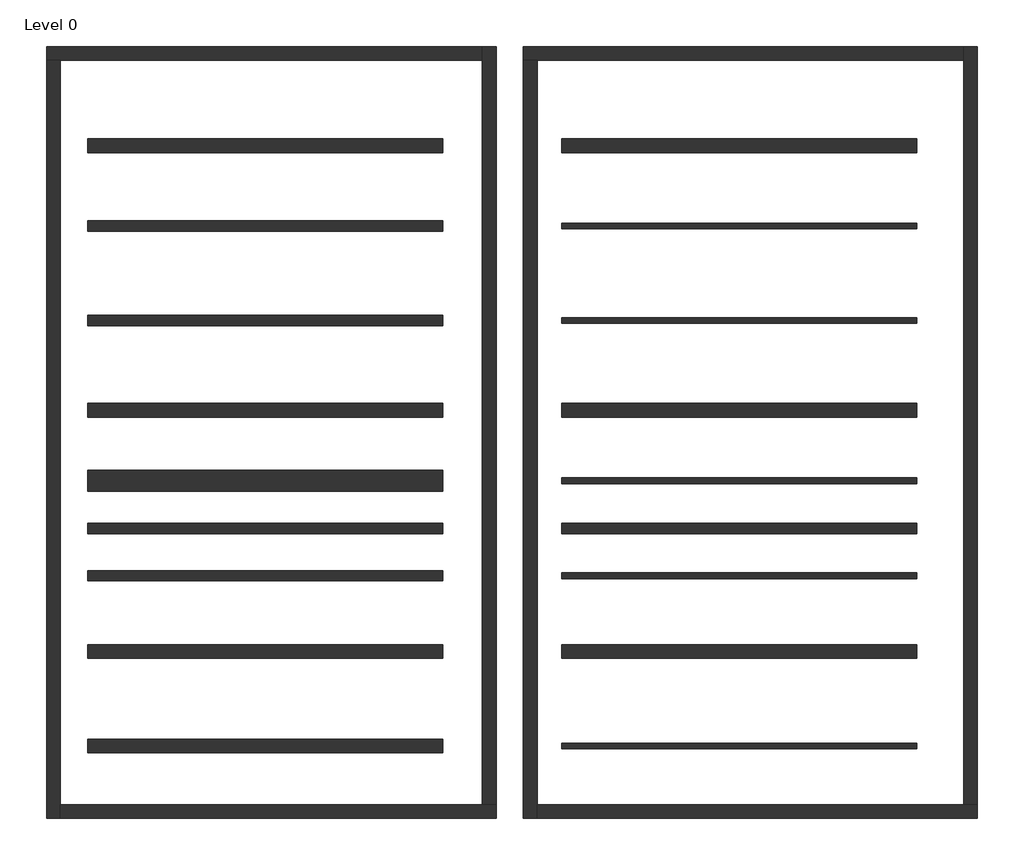
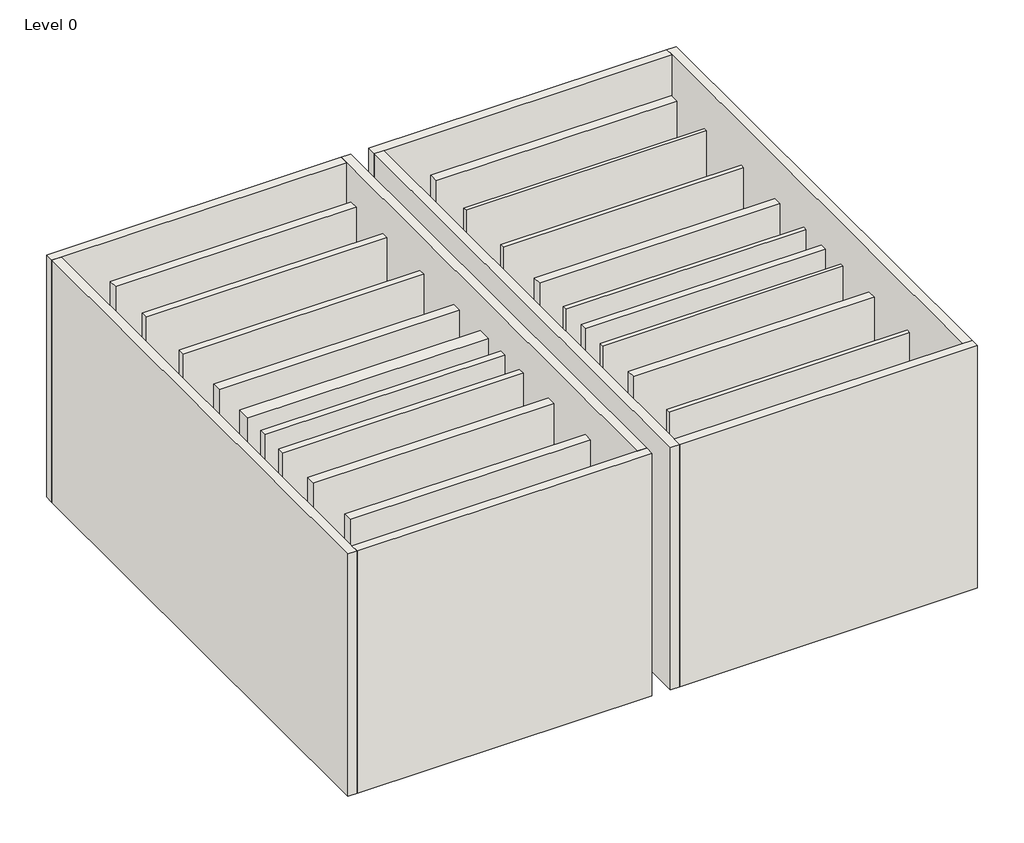
# One storey: 26 walls.
"""IFC4 building model written with IfcOpenShell, lengths in millimetres."""

from ifc_helpers import new_model, si_unit, origin, origin_with_axes, place, context, project, spatial, polyline, outline, extrude, faceted_brep, element, save

model = new_model("IFC4")

# Units and contexts
model_context = context("Model", 3, world=origin())
ifc_project = project(units=[si_unit("LENGTHUNIT", "METRE", prefix="MILLI")], contexts=[model_context])

# Site, building, storey
site = spatial("IfcSite", under=ifc_project)
building = spatial("IfcBuilding", under=site)
storey = spatial("IfcBuildingStorey", under=building, Name="Level 0", Elevation=0.0)

# Walls
placement = place(None, origin())
element("IfcWall", 1, ObjectType="Wall-Ext_102Bwk-75Ins-100LBlk-12P", at=placement, inside=storey, context=model_context, shape_type="SweptSolid", body=[
    extrude(outline(polyline([(-468.4786937, 4696.5247192), (-7968.4786937, 4696.5247192), (-7968.4786937, 4986.5247192), (-468.4786937, 4986.5247192), (-468.4786937, 4696.5247192)])), origin_with_axes(), (0.0, 0.0, 1.0), 8000.0),
])
element("IfcWall", 2, ObjectType="Wall-Ext_102Bwk-75Ins-100LBlk-12P", at=placement, inside=storey, context=model_context, shape_type="SweptSolid", body=[
    extrude(outline(polyline([(-468.4786937, -889.0752808), (-7968.4786937, -889.0752808), (-7968.4786937, -599.0752808), (-468.4786937, -599.0752808), (-468.4786937, -889.0752808)])), origin_with_axes(), (0.0, 0.0, 1.0), 8000.0),
])
element("IfcWall", 3, ObjectType="Wall-Ext_102Bwk-75Ins-100LBlk-12P", at=placement, inside=storey, context=model_context, shape_type="SweptSolid", body=[
    extrude(outline(polyline([(-468.4786937, -5979.4752808), (-7968.4786937, -5979.4752808), (-7968.4786937, -5689.4752808), (-468.4786937, -5689.4752808), (-468.4786937, -5979.4752808)])), origin_with_axes(), (0.0, 0.0, 1.0), 8000.0),
])
element("IfcWall", 4, ObjectType="Wall-Ext_102Bwk-75Ins-100LBlk-12P", at=placement, inside=storey, context=model_context, shape_type="SweptSolid", body=[
    extrude(outline(polyline([(-468.4786937, -7974.6752808), (-7968.4786937, -7974.6752808), (-7968.4786937, -7684.6752808), (-468.4786937, -7684.6752808), (-468.4786937, -7974.6752808)])), origin_with_axes(), (0.0, 0.0, 1.0), 8000.0),
])
element("IfcWall", 5, ObjectType="Wall-Ext_102Bwk-75Ins-100LBlk-12P", at=placement, inside=storey, context=model_context, shape_type="SweptSolid", body=[
    extrude(outline(polyline([(9536.3213063, 4696.5247192), (2036.3213063, 4696.5247192), (2036.3213063, 4986.5247192), (9536.3213063, 4986.5247192), (9536.3213063, 4696.5247192)])), origin_with_axes(), (0.0, 0.0, 1.0), 8000.0),
])
element("IfcWall", 6, ObjectType="Wall-Ext_102Bwk-75Ins-100LBlk-12P", at=placement, inside=storey, context=model_context, shape_type="SweptSolid", body=[
    extrude(outline(polyline([(9536.3213063, -889.0752808), (2036.3213063, -889.0752808), (2036.3213063, -599.0752808), (9536.3213063, -599.0752808), (9536.3213063, -889.0752808)])), origin_with_axes(), (0.0, 0.0, 1.0), 8000.0),
])
element("IfcWall", 7, ObjectType="Wall-Ext_102Bwk-75Ins-100LBlk-12P", at=placement, inside=storey, context=model_context, shape_type="SweptSolid", body=[
    extrude(outline(polyline([(9536.3213063, -5979.4752808), (2036.3213063, -5979.4752808), (2036.3213063, -5689.4752808), (9536.3213063, -5689.4752808), (9536.3213063, -5979.4752808)])), origin_with_axes(), (0.0, 0.0, 1.0), 8000.0),
])
element("IfcWall", 8, ObjectType="Wall-Ext_102Bwk-75Ins-100LBlk-12P", at=placement, inside=storey, context=model_context, shape_type="Brep", body=[
    faceted_brep([(-8835.7862376, 6643.8662444, 0.0), (-8545.7862376, 6643.8662444, 0.0), (364.2137624, 6643.8662444, 0.0), (364.2137624, 6643.8662444, 8000.0), (-8545.7862376, 6643.8662444, 8000.0), (-8835.7862376, 6643.8662444, 8000.0), (-8835.7862376, 6933.8662444, 0.0), (-8835.7862376, 6933.8662444, 8000.0), (364.2137624, 6933.8662444, 8000.0), (364.2137624, 6933.8662444, 0.0)], [[[0, 1, 2, 3, 4, 5]], [[6, 7, 8, 9]], [[2, 1, 0, 6, 9]], [[5, 4, 3, 8, 7]], [[0, 5, 7, 6]], [[3, 2, 9, 8]]]),
])
element("IfcWall", 9, ObjectType="Wall-Ext_102Bwk-75Ins-100LBlk-12P", at=placement, inside=storey, context=model_context, shape_type="Brep", body=[
    faceted_brep([(-8545.7862376, -9356.1337556, 0.0), (-8545.7862376, -9066.1337556, 0.0), (-8545.7862376, 6643.8662444, 0.0), (-8545.7862376, 6643.8662444, 8000.0), (-8545.7862376, -9066.1337556, 8000.0), (-8545.7862376, -9356.1337556, 8000.0), (-8835.7862376, -9356.1337556, 0.0), (-8835.7862376, -9356.1337556, 8000.0), (-8835.7862376, 6643.8662444, 8000.0), (-8835.7862376, 6643.8662444, 0.0)], [[[0, 1, 2, 3, 4, 5]], [[6, 7, 8, 9]], [[2, 1, 0, 6, 9]], [[5, 4, 3, 8, 7]], [[0, 5, 7, 6]], [[3, 2, 9, 8]]]),
])
element("IfcWall", 10, ObjectType="Wall-Ext_102Bwk-75Ins-100LBlk-12P", at=placement, inside=storey, context=model_context, shape_type="Brep", body=[
    faceted_brep([(654.2137624, -9066.1337556, 0.0), (364.2137624, -9066.1337556, 0.0), (-8545.7862376, -9066.1337556, 0.0), (-8545.7862376, -9066.1337556, 8000.0), (364.2137624, -9066.1337556, 8000.0), (654.2137624, -9066.1337556, 8000.0), (654.2137624, -9356.1337556, 0.0), (654.2137624, -9356.1337556, 8000.0), (-8545.7862376, -9356.1337556, 8000.0), (-8545.7862376, -9356.1337556, 0.0)], [[[0, 1, 2, 3, 4, 5]], [[6, 7, 8, 9]], [[2, 1, 0, 6, 9]], [[5, 4, 3, 8, 7]], [[0, 5, 7, 6]], [[3, 2, 9, 8]]]),
])
element("IfcWall", 11, ObjectType="Wall-Ext_102Bwk-75Ins-100LBlk-12P", at=placement, inside=storey, context=model_context, shape_type="Brep", body=[
    faceted_brep([(364.2137624, 6933.8662444, 0.0), (364.2137624, 6643.8662444, 0.0), (364.2137624, -9066.1337556, 0.0), (364.2137624, -9066.1337556, 8000.0), (364.2137624, 6643.8662444, 8000.0), (364.2137624, 6933.8662444, 8000.0), (654.2137624, 6933.8662444, 0.0), (654.2137624, 6933.8662444, 8000.0), (654.2137624, -9066.1337556, 8000.0), (654.2137624, -9066.1337556, 0.0)], [[[0, 1, 2, 3, 4, 5]], [[6, 7, 8, 9]], [[2, 1, 0, 6, 9]], [[5, 4, 3, 8, 7]], [[0, 5, 7, 6]], [[3, 2, 9, 8]]]),
])
element("IfcWall", 12, ObjectType="Wall-Ext_102Bwk-75Ins-100LBlk-12P", at=placement, inside=storey, context=model_context, shape_type="Brep", body=[
    faceted_brep([(1227.1253158, 6643.8662444, 0.0), (1517.1253158, 6643.8662444, 0.0), (10522.526666, 6643.8662444, 0.0), (10522.526666, 6643.8662444, 8000.0), (1517.1253158, 6643.8662444, 8000.0), (1227.1253158, 6643.8662444, 8000.0), (1227.1253158, 6933.8662444, 0.0), (1227.1253158, 6933.8662444, 8000.0), (10522.526666, 6933.8662444, 8000.0), (10522.526666, 6933.8662444, 0.0)], [[[0, 1, 2, 3, 4, 5]], [[6, 7, 8, 9]], [[2, 1, 0, 6, 9]], [[5, 4, 3, 8, 7]], [[0, 5, 7, 6]], [[3, 2, 9, 8]]]),
])
element("IfcWall", 13, ObjectType="Wall-Ext_102Bwk-75Ins-100LBlk-12P", at=placement, inside=storey, context=model_context, shape_type="Brep", body=[
    faceted_brep([(1517.1253158, -9356.1337556, 0.0), (1517.1253158, -9066.1337556, 0.0), (1517.1253158, 6643.8662444, 0.0), (1517.1253158, 6643.8662444, 8000.0), (1517.1253158, -9066.1337556, 8000.0), (1517.1253158, -9356.1337556, 8000.0), (1227.1253158, -9356.1337556, 0.0), (1227.1253158, -9356.1337556, 8000.0), (1227.1253158, 6643.8662444, 8000.0), (1227.1253158, 6643.8662444, 0.0)], [[[0, 1, 2, 3, 4, 5]], [[6, 7, 8, 9]], [[2, 1, 0, 6, 9]], [[5, 4, 3, 8, 7]], [[0, 5, 7, 6]], [[3, 2, 9, 8]]]),
])
element("IfcWall", 14, ObjectType="Wall-Ext_102Bwk-75Ins-100LBlk-12P", at=placement, inside=storey, context=model_context, shape_type="Brep", body=[
    faceted_brep([(10812.526666, -9066.1337556, 0.0), (10522.526666, -9066.1337556, 0.0), (1517.1253158, -9066.1337556, 0.0), (1517.1253158, -9066.1337556, 8000.0), (10522.526666, -9066.1337556, 8000.0), (10812.526666, -9066.1337556, 8000.0), (10812.526666, -9356.1337556, 0.0), (10812.526666, -9356.1337556, 8000.0), (1517.1253158, -9356.1337556, 8000.0), (1517.1253158, -9356.1337556, 0.0)], [[[0, 1, 2, 3, 4, 5]], [[6, 7, 8, 9]], [[2, 1, 0, 6, 9]], [[5, 4, 3, 8, 7]], [[0, 5, 7, 6]], [[3, 2, 9, 8]]]),
])
element("IfcWall", 15, ObjectType="Wall-Ext_102Bwk-75Ins-100LBlk-12P", at=placement, inside=storey, context=model_context, shape_type="Brep", body=[
    faceted_brep([(10522.526666, 6933.8662444, 0.0), (10522.526666, 6643.8662444, 0.0), (10522.526666, -9066.1337556, 0.0), (10522.526666, -9066.1337556, 8000.0), (10522.526666, 6643.8662444, 8000.0), (10522.526666, 6933.8662444, 8000.0), (10812.526666, 6933.8662444, 0.0), (10812.526666, 6933.8662444, 8000.0), (10812.526666, -9066.1337556, 8000.0), (10812.526666, -9066.1337556, 0.0)], [[[0, 1, 2, 3, 4, 5]], [[6, 7, 8, 9]], [[2, 1, 0, 6, 9]], [[5, 4, 3, 8, 7]], [[0, 5, 7, 6]], [[3, 2, 9, 8]]]),
])
element("IfcWall", 16, ObjectType="Wall-Ext_215Bwk", at=placement, inside=storey, context=model_context, shape_type="SweptSolid", body=[
    extrude(outline(polyline([(-468.4786937, 3038.8247192), (-7968.4786937, 3038.8247192), (-7968.4786937, 3253.8247192), (-468.4786937, 3253.8247192), (-468.4786937, 3038.8247192)])), origin_with_axes(), (0.0, 0.0, 1.0), 8000.0),
])
element("IfcWall", 17, ObjectType="Wall-Ext_215Bwk", at=placement, inside=storey, context=model_context, shape_type="SweptSolid", body=[
    extrude(outline(polyline([(-468.4786937, 1043.6247192), (-7968.4786937, 1043.6247192), (-7968.4786937, 1258.6247192), (-468.4786937, 1258.6247192), (-468.4786937, 1043.6247192)])), origin_with_axes(), (0.0, 0.0, 1.0), 8000.0),
])
element("IfcWall", 18, ObjectType="Wall-Ext_215Bwk", at=placement, inside=storey, context=model_context, shape_type="SweptSolid", body=[
    extrude(outline(polyline([(-468.4786937, -3346.7752808), (-7968.4786937, -3346.7752808), (-7968.4786937, -3131.7752808), (-468.4786937, -3131.7752808), (-468.4786937, -3346.7752808)])), origin_with_axes(), (0.0, 0.0, 1.0), 8000.0),
])
element("IfcWall", 19, ObjectType="Wall-Ext_215Bwk", at=placement, inside=storey, context=model_context, shape_type="SweptSolid", body=[
    extrude(outline(polyline([(-468.4786937, -4341.9752808), (-7968.4786937, -4341.9752808), (-7968.4786937, -4126.9752808), (-468.4786937, -4126.9752808), (-468.4786937, -4341.9752808)])), origin_with_axes(), (0.0, 0.0, 1.0), 8000.0),
])
element("IfcWall", 20, ObjectType="Wall-Ext_215Bwk", at=placement, inside=storey, context=model_context, shape_type="SweptSolid", body=[
    extrude(outline(polyline([(9536.3213063, -3346.7752808), (2036.3213063, -3346.7752808), (2036.3213063, -3131.7752808), (9536.3213063, -3131.7752808), (9536.3213063, -3346.7752808)])), origin_with_axes(), (0.0, 0.0, 1.0), 8000.0),
])
element("IfcWall", 21, ObjectType="Wall-Fnd_440Blk", at=placement, inside=storey, context=model_context, shape_type="SweptSolid", body=[
    extrude(outline(polyline([(-468.4786937, -2449.6752808), (-7968.4786937, -2449.6752808), (-7968.4786937, -2009.6752808), (-468.4786937, -2009.6752808), (-468.4786937, -2449.6752808)])), origin_with_axes(), (0.0, 0.0, 1.0), 8000.0),
])
element("IfcWall", 22, ObjectType="Wall-Int_12P-100Blk-12P", at=placement, inside=storey, context=model_context, shape_type="SweptSolid", body=[
    extrude(outline(polyline([(9536.3213063, 3083.8247192), (2036.3213063, 3083.8247192), (2036.3213063, 3208.8247192), (9536.3213063, 3208.8247192), (9536.3213063, 3083.8247192)])), origin_with_axes(), (0.0, 0.0, 1.0), 8000.0),
])
element("IfcWall", 23, ObjectType="Wall-Int_12P-100Blk-12P", at=placement, inside=storey, context=model_context, shape_type="SweptSolid", body=[
    extrude(outline(polyline([(9536.3213063, 1088.6247192), (2036.3213063, 1088.6247192), (2036.3213063, 1213.6247192), (9536.3213063, 1213.6247192), (9536.3213063, 1088.6247192)])), origin_with_axes(), (0.0, 0.0, 1.0), 8000.0),
])
element("IfcWall", 24, ObjectType="Wall-Int_12P-100Blk-12P", at=placement, inside=storey, context=model_context, shape_type="SweptSolid", body=[
    extrude(outline(polyline([(9536.3213063, -7892.1752808), (2036.3213063, -7892.1752808), (2036.3213063, -7767.1752808), (9536.3213063, -7767.1752808), (9536.3213063, -7892.1752808)])), origin_with_axes(), (0.0, 0.0, 1.0), 8000.0),
])
element("IfcWall", 25, ObjectType="Wall-Int_12P-100Blk-12P", at=placement, inside=storey, context=model_context, shape_type="SweptSolid", body=[
    extrude(outline(polyline([(9536.3213063, -4296.9752808), (2036.3213063, -4296.9752808), (2036.3213063, -4171.9752808), (9536.3213063, -4171.9752808), (9536.3213063, -4296.9752808)])), origin_with_axes(), (0.0, 0.0, 1.0), 8000.0),
])
element("IfcWall", 26, ObjectType="Wall-Int_12P-100Blk-12P", at=placement, inside=storey, context=model_context, shape_type="SweptSolid", body=[
    extrude(outline(polyline([(9536.3213063, -2292.1752808), (2036.3213063, -2292.1752808), (2036.3213063, -2167.1752808), (9536.3213063, -2167.1752808), (9536.3213063, -2292.1752808)])), origin_with_axes(), (0.0, 0.0, 1.0), 8000.0),
])

save(model, "model.ifc")

# Revit data of these elements
# Project information
#   Project Issue Date = "Issue Date"
#   Project Status = "Project Status"
#   Client Name = "Owner"
#   Project Address = "Enter address here"
#   Project Name = "Project Name"
#   Project Number = "Project Number"
# Type "Wall-Ext_102Bwk-75Ins-100LBlk-12P"
#   Keynote = "F10"
#   Layers, outside or top first: 102.5 mm "Brick, Common" (function 4); 75 mm "Fiberglass Batt" (function 3); 100 mm "Concrete Masonry Units _Low Density" (function 1); 12.5 mm "Plaster" (function 5)
# Type "Wall-Ext_215Bwk"
#   Keynote = "F10"
#   Layers, outside or top first: 215 mm "Brick, Common" (function 1)
# Type "Wall-Fnd_440Blk"
#   Keynote = "F10"
#   Layers, outside or top first: 440 mm "Concrete Masonry Units" (function 1)
# Type "Wall-Int_12P-100Blk-12P"
#   Layers, outside or top first: 12.5 mm "Plaster" (function 5); 100 mm "Concrete Masonry Units" (function 1); 12.5 mm "Plaster" (function 5)
# Elements 1, 2, 3, 4, 5, 6, 7 (IfcWall, "Wall-Ext_102Bwk-75Ins-100LBlk-12P")
#   Top Offset = 0 mm
#   Base Offset = 0 mm
#   Unconnected Height = 8000 mm
#   wall height = 8000 mm
#   Phase Created = New Construction
#   Base Constraint = Level 0
#   Materials on its faces: "Default Wall", "Plaster", "Brick, Common"
# Elements 8, 9, 10, 11, 12, 13, 14, 15 (IfcWall, "Wall-Ext_102Bwk-75Ins-100LBlk-12P")
#   Top Offset = 0 mm
#   Base Offset = 0 mm
#   Unconnected Height = 8000 mm
#   wall height = 8000 mm
#   Phase Created = New Construction
#   Base Constraint = Level 0
#   Materials on its faces: "Default Wall", "Brick, Common", "Plaster"
# Elements 16, 17, 18, 19, 20 (IfcWall, "Wall-Ext_215Bwk")
#   Top Offset = 0 mm
#   Base Offset = 0 mm
#   Unconnected Height = 8000 mm
#   wall height = 8000 mm
#   Phase Created = New Construction
#   Base Constraint = Level 0
#   Materials on its faces: "Brick, Common"
# Element 21 (IfcWall, "Wall-Fnd_440Blk")
#   Top Offset = 0 mm
#   Base Offset = 0 mm
#   Unconnected Height = 8000 mm
#   wall height = 8000 mm
#   Phase Created = New Construction
#   Base Constraint = Level 0
#   Materials on its faces: "Concrete Masonry Units"
# Elements 22, 23, 24, 25, 26 (IfcWall, "Wall-Int_12P-100Blk-12P")
#   Top Offset = 0 mm
#   Base Offset = 0 mm
#   Unconnected Height = 8000 mm
#   wall height = 8000 mm
#   Phase Created = New Construction
#   Base Constraint = Level 0
#   Materials on its faces: "Default Wall", "Plaster"
# Materials
#   "Brick, Common": class "Masonry", colour RGB 170 100 105, transparency 0, Description = "Common brick", Cost = 0
#   "Fiberglass Batt": class "Generic", colour RGB 127 127 127, transparency 0, Description = "Fiberglass batt insulation", Cost = 0
#   "Concrete Masonry Units _Low Density": class "Masonry", colour RGB 181 181 181, transparency 0, Description = "Concrete masonry units", Cost = 0
#   "Plaster": class "Generic", colour RGB 249 249 249, transparency 0, Description = "Plaster", Cost = 0
#   "Concrete Masonry Units": class "Masonry", colour RGB 181 181 181, transparency 0, Description = "Concrete masonry units", Cost = 0
#   "Default Wall": class "Miscellaneous", colour RGB 128 128 128, transparency 0, Comments = "Rendering appearance not upgraded ", Cost = 0
# Room at (-3446.133, 1672.132) mm, phase "New Construction", upper level "Level 0", upper offset 4000 mm, lower offset 0 mm
#   Number = "1"
#   Name = "Room"
# Room at (5763.989, 1672.132) mm, phase "New Construction", upper level "Level 0", upper offset 4000 mm, lower offset 0 mm
#   Number = "2"
#   Name = "Room"
